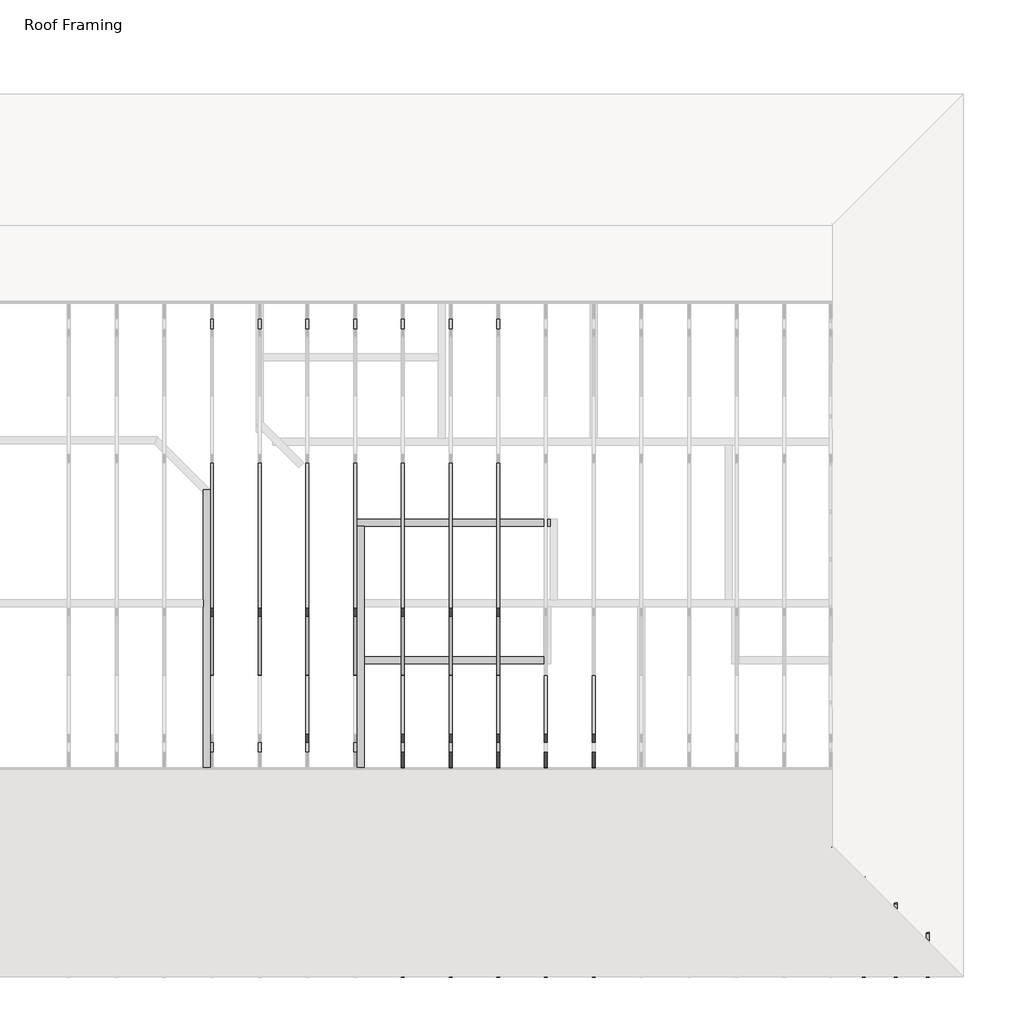
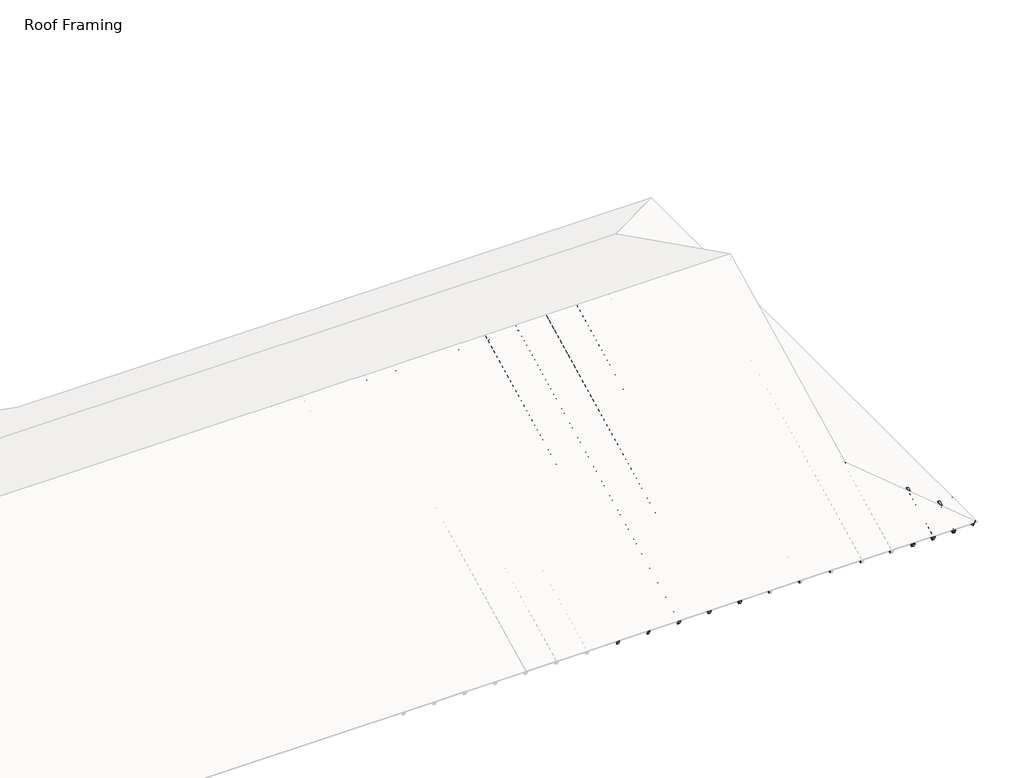
# One storey, part 3 of 7: 48 beams, 13 members.
# Revit data of these elements (continued)
# Elements 2, 5 (IfcBeam, "Dimension Lumber : Roof Lumbers") (continued)
#   Phase Created = New Construction
#   Materials on its faces: "Douglas Fir #2"
# Elements 6, 16, 17, 18, 21 (IfcBeam, "Dimension Lumber : Top Supporting Lumbers")
#   Structural Material = Douglas Fir #2
#   Phase Created = New Construction
#   Materials on its faces: "Douglas Fir #2"
# Elements 7, 8, 9, 10 (IfcBeam, "Dimension Lumber : Roof Lumbers")
#   Structural Material = Softwood, Lumber
#   Phase Created = New Construction
#   Materials on its faces: "Softwood, Lumber"
# Elements 11, 12, 13, 14, 15, 19, 20 (IfcBeam, "Dimension Lumber : Top Supporting Lumbers")
#   Comments = ""
#   Structural Material = Douglas Fir #2
#   Phase Created = New Construction
#   Materials on its faces: "Douglas Fir #2"
# Elements 22, 23, 24, 25, 26, 27, 28, 29, 30, 31, 32, 33, 34, 35, 36 (IfcBeam, "Dimension Lumber : 2x4 Blocking")
#   Comments = ""
#   Structural Material = Douglas Fir #2
#   Phase Created = New Construction
#   Materials on its faces: "Douglas Fir #2"
# Elements 37, 38, 40, 42, 44 (IfcBeam, "Dimension Lumber : 2x4 Truss")
#   Structural Material = Douglas Fir #2
#   Phase Created = New Construction
#   Materials on its faces: "Douglas Fir #2"
# Elements 39, 41, 43, 45, 46, 47, 48 (IfcBeam, "Dimension Lumber : 2x4 Truss")
#   Comments = ""
#   Structural Material = Douglas Fir #2
#   Phase Created = New Construction
#   Materials on its faces: "Douglas Fir #2"
# Elements 49, 50, 51, 52, 53, 54, 55, 56, 57, 58, 59, 60, 61 (IfcMember, "Dimension Lumber : 2x4 Truss")
#   Comments = ""
#   Structural Material = Douglas Fir #2
#   Phase Created = New Construction
#   Materials on its faces: "Douglas Fir #2"
# Materials
#   "Softwood, Lumber": class "Wood", colour RGB 223 192 134, transparency 0, Description = "Pinus Echinata", Cost = 0
#   "Douglas Fir #2": class "Wood", colour RGB 223 192 134, transparency 0, Description = "Pinus Echinata", Cost = 0
